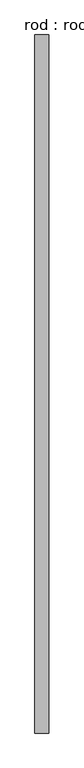
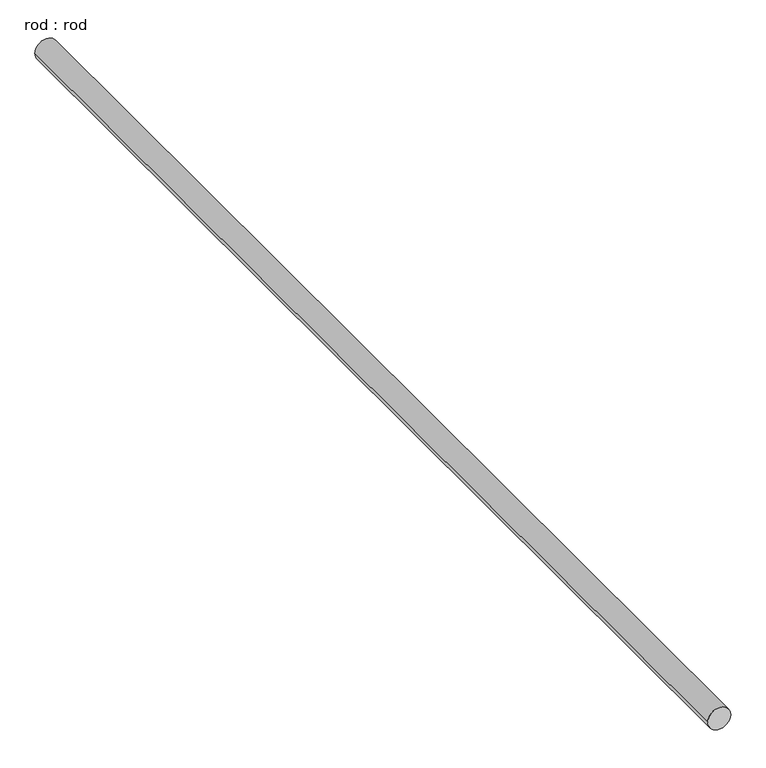
"""IFC4 building model written with IfcOpenShell, lengths in millimetres: proxy geometry, rod : rod."""

from ifc_helpers import new_model, si_unit, point, frame, frame_2d, origin, place, context, project, spatial, circle_curve, trimmed, segment, composite_curve, outline, extrude, source, transform, mapped, element, save


def rod_rod_437046fa(model_context):
    return source(origin(), model_context, "Body", "SweptSolid", [
        extrude(outline(composite_curve([segment(trimmed(circle_curve(frame_2d((0.0108462, 0.0)), 200.0), [point((0.0108462, 200.0))], [point((0.0108462, -200.0))], False, "CARTESIAN"), True, "CONTINUOUS"), segment(trimmed(circle_curve(frame_2d((0.0108462, 0.0)), 200.0), [point((0.0108462, -200.0))], [point((0.0108462, 200.0))], False, "CARTESIAN"), True, "CONTINUOUS")], self_intersect=False)), frame((0.0, -6086.1445972, 0.0), z_axis=(0.0, 1.0, 0.0), x_axis=(0.0, 0.0, 1.0)), (0.0, 0.0, 1.0), 20357.746425),
    ])


if __name__ == "__main__":
    model = new_model("IFC4")
    model_context = context("Model", 3, world=origin())
    ifc_project = project(units=[si_unit("LENGTHUNIT", "METRE", prefix="MILLI")], contexts=[model_context])
    site = spatial("IfcSite", under=ifc_project)
    building = spatial("IfcBuilding", under=site)
    placement = place(None, origin())
    rod_rod_shape = rod_rod_437046fa(model_context)
    element("IfcBuildingElementProxy", 1, Name="rod : rod", ObjectType="rod : rod", at=placement, inside=building, context=model_context, shape_type="MappedRepresentation", body=[
        mapped(rod_rod_shape, transform((0.0, 0.0, 0.0), x_axis=(1.0, 0.0, 0.0), y_axis=(0.0, 1.0, 0.0), z_axis=(0.0, 0.0, 1.0))),
    ])
    save(model, "model.ifc")

# Revit data of these elements
# Type "rod : rod"
#   Default Elevation = 0
